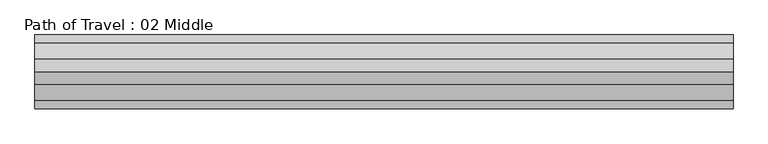
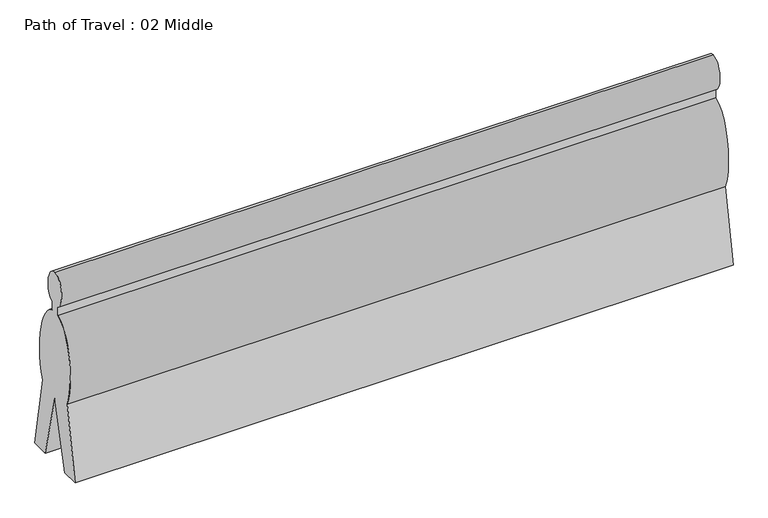
"""IFC4 building model written with IfcOpenShell, lengths in millimetres: proxy geometry, Path of Travel : 02 Middle."""

import ifcopenshell
import ifcopenshell.guid

model = None  # the IFC model being written
_history = None  # IfcOwnerHistory: only IFC2X3 demands one
_inside = {}  # id of a spatial element -> (the spatial element, [elements in it])
_under = {}  # id of a project, library or spatial element -> (it, [spatial elements below it])
_declared = {}  # id of a project -> (the project, [libraries it declares])
_typed = {}  # id of a type object -> (the type object, [elements of that type])
_made_of = {}  # id of a material, layer set ... -> (it, [elements and type objects made of it])


def new_model(schema):
    """Start an empty IFC model of exactly this schema.

    Asked for "IFC4X3", IfcOpenShell would pick the latest addendum, in which some entities
    have other attributes; the version numbers below select the first issue.
    IFC2X3 requires an IfcOwnerHistory on every rooted entity: one is made here for all.
    """
    global model, _history
    if schema == "IFC4X3":
        model = ifcopenshell.file(schema_version=(4, 3, 0, 0))
    else:
        model = ifcopenshell.file(schema=schema)
    _inside.clear()
    _under.clear()
    _declared.clear()
    _typed.clear()
    _made_of.clear()
    _history = None
    if model.schema == "IFC2X3":
        org = make("IfcOrganization", Name="unknown")
        user = make(
            "IfcPersonAndOrganization",
            ThePerson=make("IfcPerson", FamilyName="unknown"),
            TheOrganization=org,
        )
        app = make(
            "IfcApplication",
            ApplicationDeveloper=org,
            Version="unknown",
            ApplicationFullName="unknown",
            ApplicationIdentifier="unknown",
        )
        _history = make(
            "IfcOwnerHistory",
            OwningUser=user,
            OwningApplication=app,
            ChangeAction="ADDED",
            CreationDate=0,
        )
    return model


def make(cls, **values):
    """One entity of the class cls with the attributes given. An attribute that is None is left unset."""
    return model.create_entity(
        cls, **{name: value for name, value in values.items() if value is not None}
    )


def rooted(cls, **values):
    """An entity with a GlobalId (a new one), such as an element, a storey or a relation."""
    return make(cls, GlobalId=ifcopenshell.guid.new(), OwnerHistory=_history, **values)


def si_unit(unit_type, name, prefix=None):
    """IfcSIUnit, for example si_unit("LENGTHUNIT", "METRE", prefix="MILLI")."""
    return make("IfcSIUnit", UnitType=unit_type, Prefix=prefix, Name=name)


def assignment(units):
    """IfcUnitAssignment: the units of a project."""
    return None if units is None else make("IfcUnitAssignment", Units=units)


def point(xyz):
    """IfcCartesianPoint."""
    return None if xyz is None else make("IfcCartesianPoint", Coordinates=xyz)


def direction(xyz):
    """IfcDirection."""
    return None if xyz is None else make("IfcDirection", DirectionRatios=xyz)


def frame(location, z_axis=None, x_axis=None):
    """IfcAxis2Placement3D, a coordinate frame: its origin and axes. An axis left out is left unset."""
    return make(
        "IfcAxis2Placement3D",
        Location=point(location),
        Axis=direction(z_axis),
        RefDirection=direction(x_axis),
    )


def origin():
    """The frame at (0, 0, 0) with its axes left unset."""
    return frame((0.0, 0.0, 0.0))


def place(relative_to, where):
    """IfcLocalPlacement: puts the frame where relative to a parent placement (None: the world)."""
    return make(
        "IfcLocalPlacement", PlacementRelTo=relative_to, RelativePlacement=where
    )


def context(
    kind, dimensions, precision=None, world=None, true_north=None, identifier=None
):
    """IfcGeometricRepresentationContext, for example the 3D "Model" context."""
    return make(
        "IfcGeometricRepresentationContext",
        ContextIdentifier=identifier,
        ContextType=kind,
        CoordinateSpaceDimension=dimensions,
        Precision=precision,
        WorldCoordinateSystem=world,
        TrueNorth=true_north,
    )


def project(units=None, contexts=None):
    """IfcProject with its units and contexts."""
    return rooted(
        "IfcProject",
        Name="project",
        RepresentationContexts=contexts,
        UnitsInContext=assignment(units),
    )


def spatial(cls, under=None, at=None, **own):
    """A site, building, storey or space (cls), placed at a placement, below another one or the project."""
    s = rooted(cls, ObjectPlacement=at, **own)
    if under is not None:
        _under.setdefault(under.id(), (under, []))[1].append(s)
    return s


def ellipse_curve(where, semi_axis1, semi_axis2):
    """IfcEllipse in the frame where."""
    return make(
        "IfcEllipse", Position=where, SemiAxis1=semi_axis1, SemiAxis2=semi_axis2
    )


def trimmed(basis, trim1, trim2, sense, master):
    """IfcTrimmedCurve: the piece of a basis curve between two trims."""
    return make(
        "IfcTrimmedCurve",
        BasisCurve=basis,
        Trim1=trim1,
        Trim2=trim2,
        SenseAgreement=sense,
        MasterRepresentation=master,
    )


def shape(context_of_items, identifier, shape_type, items):
    """IfcShapeRepresentation: the items that make up one representation, for example the "Body"."""
    return make(
        "IfcShapeRepresentation",
        ContextOfItems=context_of_items,
        RepresentationIdentifier=identifier,
        RepresentationType=shape_type,
        Items=items,
    )


def source(mapping_origin, context_of_items, identifier, shape_type, items):
    """IfcRepresentationMap: a shape defined once, which mapped items show again and again."""
    return make(
        "IfcRepresentationMap",
        MappingOrigin=mapping_origin,
        MappedRepresentation=shape(context_of_items, identifier, shape_type, items),
    )


def transform(
    local_origin,
    x_axis=None,
    y_axis=None,
    z_axis=None,
    scale=None,
    scale2=None,
    scale3=None,
    uniform=True,
):
    """IfcCartesianTransformationOperator3D, or its non-uniform kind. x_axis, y_axis, z_axis: its Axis1, 2, 3."""
    if uniform:
        return make(
            "IfcCartesianTransformationOperator3D",
            Axis1=direction(x_axis),
            Axis2=direction(y_axis),
            LocalOrigin=point(local_origin),
            Scale=scale,
            Axis3=direction(z_axis),
        )
    return make(
        "IfcCartesianTransformationOperator3DnonUniform",
        Axis1=direction(x_axis),
        Axis2=direction(y_axis),
        LocalOrigin=point(local_origin),
        Scale=scale,
        Axis3=direction(z_axis),
        Scale2=scale2,
        Scale3=scale3,
    )


def mapped(mapping_source, mapping_target):
    """IfcMappedItem: shows the shape of a source again, moved by a transform."""
    return make(
        "IfcMappedItem", MappingSource=mapping_source, MappingTarget=mapping_target
    )


def made_of(thing, what):
    """Note that an element or type object is made of a material, layer set ...; save() writes the relation."""
    if what is not None:
        _made_of.setdefault(what.id(), (what, []))[1].append(thing)
    return thing


def element(
    cls,
    number,
    at=None,
    inside=None,
    cuts=None,
    type_object=None,
    material=None,
    context=None,
    identifier="Body",
    shape_type=None,
    held_by="IfcProductDefinitionShape",
    body=None,
    shapes=None,
    **own,
):
    """One element of the class cls, such as IfcWall. Its Tag is "e" and its number.

    at: its placement. inside: the storey or other place that contains it. cuts: it is an
    opening in that element (IfcRelVoidsElement). A single representation is given by context,
    identifier, shape_type and body (its items); several are given by shapes. held_by: the class
    of the entity that holds the representations. save() writes the other relations.
    """
    e = rooted(cls, Tag="e%d" % number, ObjectPlacement=at, **own)
    if body is not None:
        shapes = [shape(context, identifier, shape_type, body)]
    if shapes is not None:
        e.Representation = make(held_by, Representations=shapes)
    if inside is not None:
        _inside.setdefault(inside.id(), (inside, []))[1].append(e)
    if cuts is not None:
        rooted(
            "IfcRelVoidsElement", RelatingBuildingElement=cuts, RelatedOpeningElement=e
        )
    if type_object is not None:
        _typed.setdefault(type_object.id(), (type_object, []))[1].append(e)
    return made_of(e, material)


def aggregate(whole, parts):
    """IfcRelAggregates: a whole, such as a stair, and the parts it consists of."""
    return rooted("IfcRelAggregates", RelatingObject=whole, RelatedObjects=parts)


def save(model, path):
    """Write the relations noted so far, then the file.

    IfcRelAggregates (storeys below a building ...), IfcRelContainedInSpatialStructure (elements
    in a storey), IfcRelDefinesByType, IfcRelAssociatesMaterial and IfcRelDeclares: one each for
    every whole, place, type object, material and project.
    """
    for whole, parts in _under.values():
        aggregate(whole, parts)
    for where, things in _inside.values():
        rooted(
            "IfcRelContainedInSpatialStructure",
            RelatedElements=things,
            RelatingStructure=where,
        )
    for kind, things in _typed.values():
        rooted("IfcRelDefinesByType", RelatedObjects=things, RelatingType=kind)
    for what, things in _made_of.values():
        rooted("IfcRelAssociatesMaterial", RelatedObjects=things, RelatingMaterial=what)
    for by, libraries in _declared.values():
        rooted("IfcRelDeclares", RelatingContext=by, RelatedDefinitions=libraries)
    model.write(path)


def plane_surface(at):
    """IfcPlane: the flat surface through the origin of the frame at, square to its z axis."""
    return make("IfcPlane", Position=at)


def extruded_surface(curve, direction_of_extrusion, depth):
    """IfcSurfaceOfLinearExtrusion: the curve pushed along a direction by depth."""
    return make(
        "IfcSurfaceOfLinearExtrusion",
        SweptCurve=make("IfcArbitraryOpenProfileDef", ProfileType="CURVE", Curve=curve),
        ExtrudedDirection=direction(direction_of_extrusion),
        Depth=depth,
    )


def advanced_brep(points, edges, surfaces, faces):
    """IfcAdvancedBrep: a solid bounded by faces that lie on surfaces and meet in shared edges.

    An edge is (start, end): straight between two places in points (the first is 0);
    or (start, end, curve); or (start, end, curve, False) where it runs against its curve.
    A face is (place in surfaces, loops), or (place, loops, False) where it looks against
    its surface's normal. A loop lists edges by number (the first is 1), with a minus sign
    where the edge is run from its end to its start. The first loop is the outer one.
    """
    corners = [point(p) for p in points]
    vertices = [make("IfcVertexPoint", VertexGeometry=c) for c in corners]
    made = []
    for start, end, *more in edges:
        made.append(
            make(
                "IfcEdgeCurve",
                EdgeStart=vertices[start],
                EdgeEnd=vertices[end],
                EdgeGeometry=more[0] if more else make("IfcPolyline", Points=[corners[start], corners[end]]),
                SameSense=more[1] if len(more) > 1 else True,
            )
        )
    hull = []
    for where, loops, *sense in faces:
        bounds = []
        for j, loop in enumerate(loops):
            ring = [make("IfcOrientedEdge", EdgeElement=made[abs(k) - 1], Orientation=k > 0) for k in loop]
            bounds.append(
                make(
                    "IfcFaceOuterBound" if j == 0 else "IfcFaceBound",
                    Bound=make("IfcEdgeLoop", EdgeList=ring),
                    Orientation=True,
                )
            )
        hull.append(make("IfcAdvancedFace", Bounds=bounds, FaceSurface=surfaces[where], SameSense=sense[0] if sense else True))
    return make("IfcAdvancedBrep", Outer=make("IfcClosedShell", CfsFaces=hull))


def path_of_travel_02_middle_da6d7806(model_context):
    return source(origin(), model_context, "Body", "AdvancedBrep", [
        advanced_brep(
        [(227.5554837, 0.0, 1727.2), (227.5554837, 42.9018657, 1436.6534209), (227.5554837, 42.9018657, 1363.4763406), (227.5554837, 184.1186263, 643.4144547), (227.5554837, 297.5699544, 0.0), (227.5554837, 145.6574193, 0.0), (227.5554837, 0.0, 584.2), (227.5554837, -145.6574193, 0.0), (227.5554837, -297.5699544, 0.0), (227.5554837, -184.1186263, 643.4144547), (227.5554837, -42.9018657, 1363.4763406), (227.5554837, -42.9018657, 1436.6534209), (5866.3554837, 0.0, 1727.2), (5866.3554837, -42.9018657, 1436.6534209), (5866.3554837, -42.9018657, 1363.4763406), (5866.3554837, -184.1186263, 643.4144547), (5866.3554837, -297.5699544, 0.0), (5866.3554837, -145.6574193, 0.0), (5866.3554837, 0.0, 584.2), (5866.3554837, 145.6574193, 0.0), (5866.3554837, 297.5699544, 0.0), (5866.3554837, 184.1186263, 643.4144547), (5866.3554837, 42.9018657, 1363.4763406), (5866.3554837, 42.9018657, 1436.6534209)],
        [
            (0, 1, ellipse_curve(frame((227.5554837, 0.0, 1574.8), z_axis=(-1.0, 0.0, 0.0), x_axis=(0.0, 0.0, 1.0)), 152.4, 101.6)),
            (1, 2),
            (2, 3, ellipse_curve(frame((227.5554837, 0.0, 914.4), z_axis=(-1.0, 0.0, 0.0), x_axis=(0.0, 0.0, -1.0)), 457.2, 228.6)),
            (3, 4),
            (4, 5),
            (5, 6),
            (6, 7),
            (7, 8),
            (8, 9),
            (9, 10, ellipse_curve(frame((227.5554837, 0.0, 914.4), z_axis=(-1.0, 0.0, 0.0), x_axis=(0.0, 0.0, -1.0)), 457.2, 228.6)),
            (10, 11),
            (11, 0, ellipse_curve(frame((227.5554837, 0.0, 1574.8), z_axis=(-1.0, 0.0, 0.0), x_axis=(0.0, 0.0, 1.0)), 152.4, 101.6)),
            (12, 13, ellipse_curve(frame((5866.3554837, 0.0, 1574.8), z_axis=(1.0, 0.0, 0.0), x_axis=(0.0, 0.0, 1.0)), 152.4, 101.6)),
            (13, 14),
            (14, 15, ellipse_curve(frame((5866.3554837, 0.0, 914.4), z_axis=(1.0, 0.0, 0.0), x_axis=(0.0, 0.0, -1.0)), 457.2, 228.6)),
            (15, 16),
            (16, 17),
            (17, 18),
            (18, 19),
            (19, 20),
            (20, 21),
            (21, 22, ellipse_curve(frame((5866.3554837, 0.0, 914.4), z_axis=(1.0, 0.0, 0.0), x_axis=(0.0, 0.0, -1.0)), 457.2, 228.6)),
            (22, 23),
            (23, 12, ellipse_curve(frame((5866.3554837, 0.0, 1574.8), z_axis=(1.0, 0.0, 0.0), x_axis=(0.0, 0.0, 1.0)), 152.4, 101.6)),
            (0, 12),
            (23, 1),
            (22, 2),
            (21, 3),
            (20, 4),
            (19, 5),
            (18, 6),
            (17, 7),
            (16, 8),
            (15, 9),
            (14, 10),
            (13, 11),
        ],
        [
            plane_surface(frame((227.5554837, 0.0, 0.0), z_axis=(-1.0, 0.0, 0.0), x_axis=(0.0, 0.0, 1.0))),
            plane_surface(frame((5866.3554837, 0.0, 0.0), z_axis=(1.0, 0.0, 0.0), x_axis=(0.0, 0.0, 1.0))),
            extruded_surface(trimmed(ellipse_curve(frame((5866.3554837, 0.0, 1574.8), z_axis=(-1.0, 0.0, 0.0), x_axis=(0.0, 0.0, 1.0)), 152.4, 101.6), [point((5866.3554837, 0.0, 1727.2))], [point((5866.3554837, 42.9018657, 1436.6534209))], True, "CARTESIAN"), (-5638.8, 0.0, 0.0), 5638.8),
            plane_surface(frame((227.5554837, 42.9018657, 1436.6534209), z_axis=(0.0, 1.0, 0.0), x_axis=(1.0, 0.0, 0.0))),
            extruded_surface(trimmed(ellipse_curve(frame((5866.3554837, 0.0, 914.4), z_axis=(-1.0, 0.0, 0.0), x_axis=(0.0, 0.0, -1.0)), 457.2, 228.6), [point((5866.3554837, 42.9018657, 1363.4763406))], [point((5866.3554837, 184.1186263, 643.4144547))], True, "CARTESIAN"), (-5638.8, 0.0, 0.0), 5638.8),
            plane_surface(frame((227.5554837, 184.1186263, 643.4144547), z_axis=(0.0, 0.9848077530122078, 0.17364817766693205), x_axis=(1.0, 0.0, 0.0))),
            plane_surface(frame((227.5554837, 297.5699544, 0.0), z_axis=(0.0, 0.0, -1.0), x_axis=(1.0, 0.0, 0.0))),
            plane_surface(frame((227.5554837, 145.6574193, 0.0), z_axis=(0.0, -0.9702957262760199, -0.2419218955995739), x_axis=(1.0, 0.0, 0.0))),
            plane_surface(frame((227.5554837, 0.0, 584.2), z_axis=(0.0, 0.9702957262759961, -0.24192189559966923), x_axis=(1.0, 0.0, 0.0))),
            plane_surface(frame((227.5554837, -145.6574193, 0.0), z_axis=(0.0, 0.0, -1.0), x_axis=(1.0, 0.0, 0.0))),
            plane_surface(frame((227.5554837, -297.5699544, 0.0), z_axis=(0.0, -0.984807753012208, 0.17364817766693066), x_axis=(1.0, 0.0, 0.0))),
            extruded_surface(trimmed(ellipse_curve(frame((5866.3554837, 0.0, 914.4), z_axis=(-1.0, 0.0, 0.0), x_axis=(0.0, 0.0, -1.0)), 457.2, 228.6), [point((5866.3554837, -184.1186263, 643.4144547))], [point((5866.3554837, -42.9018657, 1363.4763406))], True, "CARTESIAN"), (-5638.8, 0.0, 0.0), 5638.8),
            plane_surface(frame((227.5554837, -42.9018657, 1363.4763406), z_axis=(0.0, -1.0, 0.0), x_axis=(1.0, 0.0, 0.0))),
            extruded_surface(trimmed(ellipse_curve(frame((5866.3554837, 0.0, 1574.8), z_axis=(-1.0, 0.0, 0.0), x_axis=(0.0, 0.0, 1.0)), 152.4, 101.6), [point((5866.3554837, -42.9018657, 1436.6534209))], [point((5866.3554837, 0.0, 1727.2))], True, "CARTESIAN"), (-5638.8, 0.0, 0.0), 5638.8),
        ],
        [
            (0, [[1, 2, 3, 4, 5, 6, 7, 8, 9, 10, 11, 12]]),
            (1, [[13, 14, 15, 16, 17, 18, 19, 20, 21, 22, 23, 24]]),
            (2, [[-1, 25, -24, 26]]),
            (3, [[-2, -26, -23, 27]]),
            (4, [[-3, -27, -22, 28]]),
            (5, [[-4, -28, -21, 29]]),
            (6, [[-5, -29, -20, 30]]),
            (7, [[-6, -30, -19, 31]]),
            (8, [[-7, -31, -18, 32]]),
            (9, [[-8, -32, -17, 33]]),
            (10, [[-9, -33, -16, 34]]),
            (11, [[-10, -34, -15, 35]]),
            (12, [[-11, -35, -14, 36]]),
            (13, [[-12, -36, -13, -25]]),
        ],
    ),
    ])


if __name__ == "__main__":
    model = new_model("IFC4")
    model_context = context("Model", 3, world=origin())
    ifc_project = project(units=[si_unit("LENGTHUNIT", "METRE", prefix="MILLI")], contexts=[model_context])
    site = spatial("IfcSite", under=ifc_project)
    building = spatial("IfcBuilding", under=site)
    placement = place(None, origin())
    path_of_travel_02_middle_shape = path_of_travel_02_middle_da6d7806(model_context)
    element("IfcBuildingElementProxy", 1, Name="Path of Travel : 02 Middle", ObjectType="Path of Travel : 02 Middle", at=placement, inside=building, context=model_context, shape_type="MappedRepresentation", body=[
        mapped(path_of_travel_02_middle_shape, transform((0.0, 0.0, 0.0), x_axis=(1.0, 0.0, 0.0), y_axis=(0.0, 1.0, 0.0), z_axis=(0.0, 0.0, 1.0))),
    ])
    save(model, "model.ifc")

# Revit data of these elements
# Type "Path of Travel : 02 Middle"
#   Path of Egress [instance default] = 4' - 0"
#   built-in parameter 1001306 [instance default] = 4 (stored number, unit not read)
#   Dot at Start = no
#   Arrow in Middle = yes
#   Arrow at End = no
#   Egress Path = none
# Element 1 (IfcBuildingElementProxy, "Path of Travel : 02 Middle")
#   Path of Egress = 18' - 6"
#   built-in parameter 1001306 = 18.5 (stored number, unit not read)
#   Materials on its faces: "Egress Path Solid"
# Materials
#   "Egress Path Solid": class "Unassigned", colour RGB 255 128 64, transparency 0.75, Comments = "Rendering appearance not upgraded "
